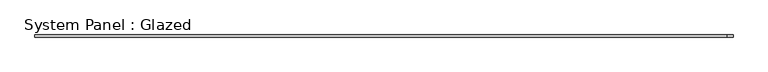
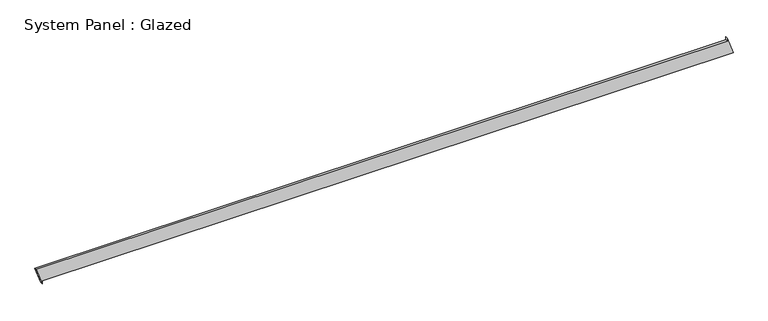
"""IFC4 building model written with IfcOpenShell, lengths in millimetres: plate geometry, System Panel : Glazed."""

from ifc_helpers import new_model, si_unit, frame, origin, place, context, project, spatial, polyline, outline, extrude, source, transform, mapped, element, save


def system_panel_glazed_77a67aa9(model_context):
    return source(origin(), model_context, "Body", "SweptSolid", [
        extrude(outline(polyline([(0.0, -3957.4553629), (35.3553391, -3957.4553629), (35.3553391, 4027.1832678), (235.4605257, 3957.794267), (200.1051866, 3957.7948933), (199.9637313, -4027.1832678), (0.0, -3957.4553629)])), frame((0.0, -49.5, 0.0), z_axis=(0.0, 1.0, 0.0), x_axis=(0.0, 0.0, 1.0)), (0.0, 0.0, 1.0), 25.0),
    ])


if __name__ == "__main__":
    model = new_model("IFC4")
    model_context = context("Model", 3, world=origin())
    ifc_project = project(units=[si_unit("LENGTHUNIT", "METRE", prefix="MILLI")], contexts=[model_context])
    site = spatial("IfcSite", under=ifc_project)
    building = spatial("IfcBuilding", under=site)
    placement = place(None, origin())
    system_panel_glazed_shape = system_panel_glazed_77a67aa9(model_context)
    element("IfcPlate", 1, ObjectType="System Panel : Glazed", at=placement, inside=building, context=model_context, shape_type="MappedRepresentation", body=[
        mapped(system_panel_glazed_shape, transform((0.0, 0.0, 0.0), x_axis=(1.0, 0.0, 0.0), y_axis=(0.0, 1.0, 0.0), z_axis=(0.0, 0.0, 1.0))),
    ])
    save(model, "model.ifc")

# Revit data of these elements
# Element 1 (IfcPlate, "System Panel : Glazed")
#   Materials on its faces: "Glass"
# Materials
#   "Glass": class "Glass", colour RGB 218 227 224, transparency 0.85, Description = "Soda Lime Glass", Cost = 0
